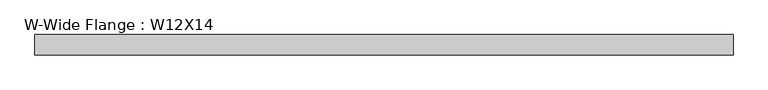
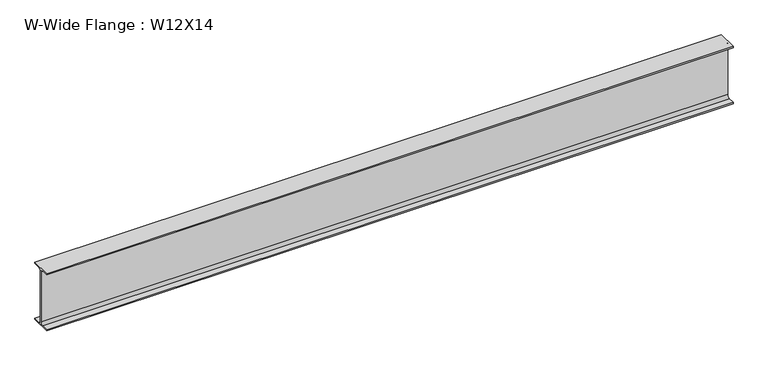
"""IFC4 building model written with IfcOpenShell, lengths in millimetres: beam geometry, W-Wide Flange : W12X14."""

from ifc_helpers import new_model, si_unit, point, frame, frame_2d, origin, place, context, project, spatial, polyline, circle_curve, trimmed, segment, composite_curve, outline, extrude, source, transform, mapped, element, save


def w_wide_flange_w12x14_48611195(model_context):
    return source(origin(), model_context, "Body", "SweptSolid", [
        extrude(outline(composite_curve([segment(polyline([(50.419, -145.415), (50.419, -151.13), (-50.419, -151.13), (-50.419, -145.415), (-15.875, -145.415)]), True, "CONTINUOUS"), segment(trimmed(circle_curve(frame_2d((-15.875, -132.08)), 13.335), [point((-15.875, -145.415))], [point((-2.54, -132.08))], True, "CARTESIAN"), True, "CONTINUOUS"), segment(polyline([(-2.54, -132.08), (-2.54, 132.08)]), True, "CONTINUOUS"), segment(trimmed(circle_curve(frame_2d((-15.875, 132.08)), 13.335), [point((-2.54, 132.08))], [point((-15.875, 145.415))], True, "CARTESIAN"), True, "CONTINUOUS"), segment(polyline([(-15.875, 145.415), (-50.419, 145.415), (-50.419, 151.13), (50.419, 151.13), (50.419, 145.415), (15.875, 145.415)]), True, "CONTINUOUS"), segment(trimmed(circle_curve(frame_2d((15.875, 132.08)), 13.335), [point((15.875, 145.415))], [point((2.54, 132.08))], True, "CARTESIAN"), True, "CONTINUOUS"), segment(polyline([(2.54, 132.08), (2.54, -132.08)]), True, "CONTINUOUS"), segment(trimmed(circle_curve(frame_2d((15.875, -132.08)), 13.335), [point((2.54, -132.08))], [point((15.875, -145.415))], True, "CARTESIAN"), True, "CONTINUOUS"), segment(polyline([(15.875, -145.415), (50.419, -145.415)]), True, "CONTINUOUS")], self_intersect=False)), frame((-1709.801, 0.0, 0.0), z_axis=(1.0, 0.0, 0.0), x_axis=(0.0, 1.0, 0.0)), (0.0, 0.0, 1.0), 3437.001),
    ])


if __name__ == "__main__":
    model = new_model("IFC4")
    model_context = context("Model", 3, world=origin())
    ifc_project = project(units=[si_unit("LENGTHUNIT", "METRE", prefix="MILLI")], contexts=[model_context])
    site = spatial("IfcSite", under=ifc_project)
    building = spatial("IfcBuilding", under=site)
    placement = place(None, origin())
    w_wide_flange_w12x14_shape = w_wide_flange_w12x14_48611195(model_context)
    element("IfcBeam", 1, ObjectType="W-Wide Flange : W12X14", at=placement, inside=building, context=model_context, shape_type="MappedRepresentation", body=[
        mapped(w_wide_flange_w12x14_shape, transform((0.0, 0.0, 0.0), x_axis=(1.0, 0.0, 0.0), y_axis=(0.0, 1.0, 0.0), z_axis=(0.0, 0.0, 1.0))),
    ])
    save(model, "model.ifc")

# Revit data of these elements
# Type "W-Wide Flange : W12X14"
#   Assembly Code = "B10"
#   W = 14
#   Length [instance default] = 5' - 0"
#   bf = 0' - 3.97"
#   d = 0' - 11.9"
#   k = 0' - 0 3/4"
#   k2 = 0' - 0.525"
#   tf = 0' - 0.225"
#   tw = 0' - 0.2"
#   A = 0.0288889 SF
#   Structural Material [instance default] = Steel ASTM A992
# Element 1 (IfcBeam, "W-Wide Flange : W12X14")
#   Materials on its faces: "Steel ASTM A992"
# Materials
#   "Steel ASTM A992": class "Metal", colour RGB 199 199 199, transparency 0, Description = "Structural steel 50ksi", Cost = 0
